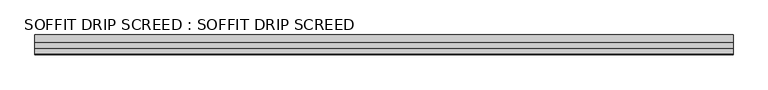
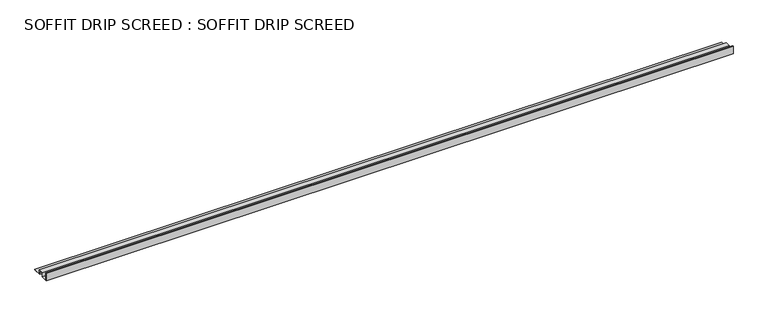
"""IFC4 building model written with IfcOpenShell, lengths in millimetres: proxy geometry, SOFFIT DRIP SCREED : SOFFIT DRIP SCREED."""

from ifc_helpers import new_model, si_unit, frame, origin, place, context, project, spatial, polyline, outline, extrude, source, transform, mapped, element, save


def soffit_drip_screed_soffit_drip_screed_d8657bfe(model_context):
    return source(origin(), model_context, "Body", "SweptSolid", [
        extrude(outline(polyline([(-5522.8747835, 39553.8960938), (-5546.5879675, 39553.8960938), (-5546.5879675, 39565.3260938), (-5559.2879675, 39565.3260938), (-5559.2879675, 39553.8960938), (-5579.8005111, 39553.8960938), (-5579.8005111, 39577.6968553), (-5578.5205111, 39577.6968553), (-5578.5205111, 39555.1760938), (-5560.5679675, 39555.1760938), (-5560.5679675, 39566.6060938), (-5545.3079675, 39566.6060938), (-5545.3079675, 39555.1760938), (-5522.8747835, 39555.1760938), (-5522.8747835, 39553.8960938)])), frame((12382.7678845, 0.0, 0.0), z_axis=(1.0, 0.0, 0.0), x_axis=(0.0, 1.0, 0.0)), (0.0, 0.0, 1.0), 2000.25),
    ])


if __name__ == "__main__":
    model = new_model("IFC4")
    model_context = context("Model", 3, world=origin())
    ifc_project = project(units=[si_unit("LENGTHUNIT", "METRE", prefix="MILLI")], contexts=[model_context])
    site = spatial("IfcSite", under=ifc_project)
    building = spatial("IfcBuilding", under=site)
    placement = place(None, origin())
    soffit_drip_screed_soffit_drip_screed_shape = soffit_drip_screed_soffit_drip_screed_d8657bfe(model_context)
    element("IfcBuildingElementProxy", 1, Name="SOFFIT DRIP SCREED : SOFFIT DRIP SCREED", ObjectType="SOFFIT DRIP SCREED : SOFFIT DRIP SCREED", at=placement, inside=building, context=model_context, shape_type="MappedRepresentation", body=[
        mapped(soffit_drip_screed_soffit_drip_screed_shape, transform((0.0, 0.0, 0.0), x_axis=(1.0, 0.0, 0.0), y_axis=(0.0, 1.0, 0.0), z_axis=(0.0, 0.0, 1.0))),
    ])
    save(model, "model.ifc")

# Revit data of these elements
# Type "SOFFIT DRIP SCREED : SOFFIT DRIP SCREED"
#   NameOverride = "SOFFIT DRIP SCREED"
# Element 1 (IfcBuildingElementProxy, "SOFFIT DRIP SCREED : SOFFIT DRIP SCREED")
#   Materials on its faces: "16 GA. COPPER VENTED SOFFIT DRIP SCREED"
# Materials
#   "16 GA. COPPER VENTED SOFFIT DRIP SCREED": class "Unassigned", colour RGB 85 255 127, transparency 0
